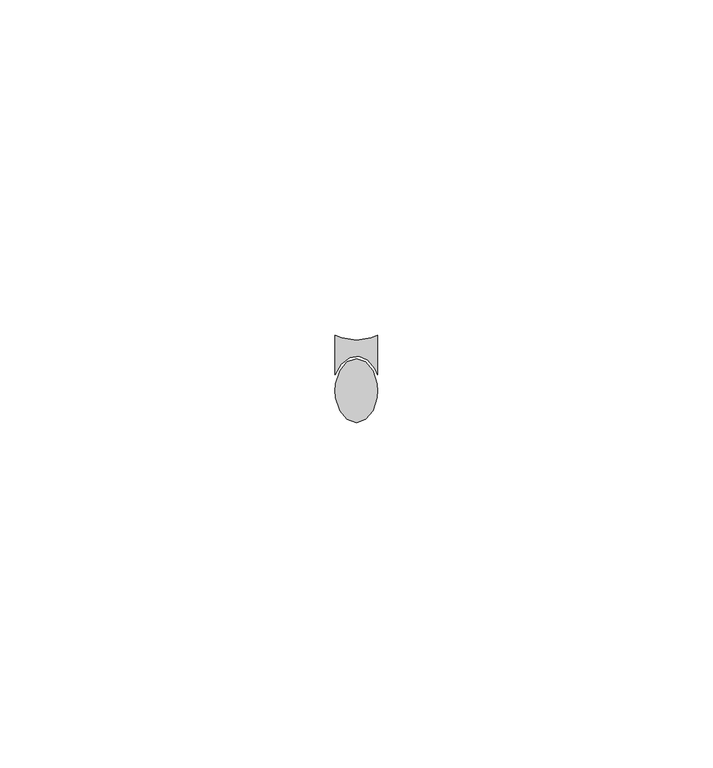
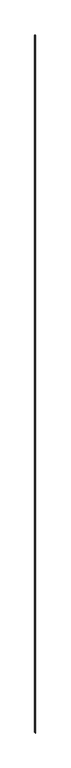
"""IFC4 building model written with IfcOpenShell, lengths in millimetres: proxy geometry, Generic Models 11:Generic Models 1:306267:Generic Models 1:306267 : Generic Models 11:Generic Models 1:306267:300405:Generic Models 1:306267:Generic Models 1:306267 : Generic Models 11:Generic Models 1:306267:300405 : Generic Models 11:Generic Models 1:306267:Generic Models 1:306267 : Generic Models 11:Generic Models 1:306267:300405:14 : Generic Models 11:Generic Models 1:306267:Generic Models 1:306267 : Generic Models 11:Generic Models 1:306267:300405:Generic Models 1:306267:Generic Models 1:306267 : Generic Models 11:Generic Models 1:306267:300405 : Generic Models 11:Generic Models 1:306267:Generic Models 1:306267 : Generic Models 11:Generic Models 1:306267:300405:300182."""

from ifc_helpers import new_model, si_unit, origin, origin_with_axes, place, context, project, spatial, polyline, outline, extrude, source, transform, mapped, element, save


def generic_models_c2f9e73e(model_context):
    return source(origin(), model_context, "Body", "SweptSolid", [
        extrude(outline(polyline([(667547.8021471, -568191.1780035), (667548.9068812, -568192.4994975), (667549.5199624, -568194.4091118), (667549.5995663, -568195.4688677), (667549.5199624, -568196.5286237), (667548.9068812, -568198.4382379), (667547.8021471, -568199.7597319), (667546.4245663, -568200.2313677), (667545.0469854, -568199.7597319), (667543.9422513, -568198.4382379), (667543.3291701, -568196.5286237), (667543.2495663, -568195.4688677), (667543.3291701, -568194.4091118), (667543.9422513, -568192.4994975), (667545.0469854, -568191.1780035), (667546.4245663, -568190.7063677), (667547.8021471, -568191.1780035)])), origin_with_axes(), (0.0, 0.0, 1.0), 8578.6515625),
        extrude(outline(polyline([(667544.2153295, -568187.6145566), (667546.4245663, -568187.9282427), (667548.633803, -568187.6145566), (667549.5995663, -568187.237148), (667549.5995663, -568193.1052401), (667549.2132487, -568192.2449592), (667548.1297632, -568190.935384), (667546.7795155, -568190.3350305), (667545.3737392, -568190.5378184), (667544.1323551, -568191.5120234), (667543.2495663, -568193.1052401), (667543.2495663, -568187.237148), (667544.2153295, -568187.6145566)])), origin_with_axes(), (0.0, 0.0, 1.0), 8578.6515625),
    ])


if __name__ == "__main__":
    model = new_model("IFC4")
    model_context = context("Model", 3, world=origin())
    ifc_project = project(units=[si_unit("LENGTHUNIT", "METRE", prefix="MILLI")], contexts=[model_context])
    site = spatial("IfcSite", under=ifc_project)
    building = spatial("IfcBuilding", under=site)
    placement = place(None, origin())
    generic_models_shape = generic_models_c2f9e73e(model_context)
    element("IfcBuildingElementProxy", 1, Name="Generic Models 11:Generic Models 1:306267:Generic Models 1:306267 : Generic Models 11:Generic Models 1:306267:300405:Generic Models 1:306267:Generic Models 1:306267 : Generic Models 11:Generic Models 1:306267:300405 : Generic Models 11:Generic Models 1:306267:Generic Models 1:306267 : Generic Models 11:Generic Models 1:306267:300405:14 : Generic Models 11:Generic Models 1:306267:Generic Models 1:306267 : Generic Models 11:Generic Models 1:306267:300405:Generic Models 1:306267:Generic Models 1:306267 : Generic Models 11:Generic Models 1:306267:300405 : Generic Models 11:Generic Models 1:306267:Generic Models 1:306267 : Generic Models 11:Generic Models 1:306267:300405:300182", ObjectType="Generic Models 11:Generic Models 1:306267:Generic Models 1:306267 : Generic Models 11:Generic Models 1:306267:300405:Generic Models 1:306267:Generic Models 1:306267 : Generic Models 11:Generic Models 1:306267:300405 : Generic Models 11:Generic Models 1:306267:Generic Models 1:306267 : Generic Models 11:Generic Models 1:306267:300405:14 : Generic Models 11:Generic Models 1:306267:Generic Models 1:306267 : Generic Models 11:Generic Models 1:306267:300405:Generic Models 1:306267:Generic Models 1:306267 : Generic Models 11:Generic Models 1:306267:300405 : Generic Models 11:Generic Models 1:306267:Generic Models 1:306267 : Generic Models 11:Generic Models 1:306267:300405:300182", at=placement, inside=building, context=model_context, shape_type="MappedRepresentation", body=[
        mapped(generic_models_shape, transform((0.0, 0.0, 0.0), x_axis=(1.0, 0.0, 0.0), y_axis=(0.0, 1.0, 0.0), z_axis=(0.0, 0.0, 1.0))),
    ])
    save(model, "model.ifc")

# Revit data of these elements
# Type "Generic Models 11:Generic Models 1:306267:Generic Models 1:306267 : Generic Models 11:Generic Models 1:306267:300405:Generic Models 1:306267:Generic Models 1:306267 : Generic Models 11:Generic Models 1:306267:300405 : Generic Models 11:Generic Models 1:306267:Generic Models 1:306267 : Generic Models 11:Generic Models 1:306267:300405:14 : Generic Models 11:Generic Models 1:306267:Generic Models 1:306267 : Generic Models 11:Generic Models 1:306267:300405:Generic Models 1:306267:Generic Models 1:306267 : Generic Models 11:Generic Models 1:306267:300405 : Generic Models 11:Generic Models 1:306267:Generic Models 1:306267 : Generic Models 11:Generic Models 1:306267:300405:300182"
#   NameOverride = "Generic Models 11:Generic Models 1:306267:Generic Models 1:306267 : Generic Models 11:Generic Models 1:306267:300405:Generic Models 1:306267:Generic Models 1:306267 : Generic Models 11:Generic Models 1:306267:300405 : Generic Models 11:Generic Models 1:306267:Generic Models 1:306267 : Generic Models 11:Generic Models 1:306267:300405:300182"
#   ObjectTypeOverride = "Generic Models 1:306267:Generic Models 1:306267 : Generic Models 11:Generic Models 1:306267:300405 : Generic Models 11:Generic Models 1:306267:Generic Models 1:306267 : Generic Models 11:Generic Models 1:306267:300405"
#   Reference = "Generic Models 1"
#   Tag = "300182"
# Element 1 (IfcBuildingElementProxy, "Generic Models 11:Generic Models 1:306267:Generic Models 1:306267 : Generic Models 11:Generic Models 1:306267:300405:Generic Models 1:306267:Generic Models 1:306267 : Generic Models 11:Generic Models 1:306267:300405 : Generic Models 11:Generic Models 1:306267:Generic Models 1:306267 : Generic Models 11:Generic Models 1:306267:300405:14 : Generic Models 11:Generic Models 1:306267:Generic Models 1:306267 : Generic Models 11:Generic Models 1:306267:300405:Generic Models 1:306267:Generic Models 1:306267 : Generic Models 11:Generic Models 1:306267:300405 : Generic Models 11:Generic Models 1:306267:Generic Models 1:306267 : Generic Models 11:Generic Models 1:306267:300405:300182")
#   Materials on its faces: "SEALANT & BACKER ROD, IF NECESSARY"
# Materials
#   "SEALANT & BACKER ROD, IF NECESSARY": class "Unassigned", colour RGB 120 120 120, transparency 0, Cost = 0
